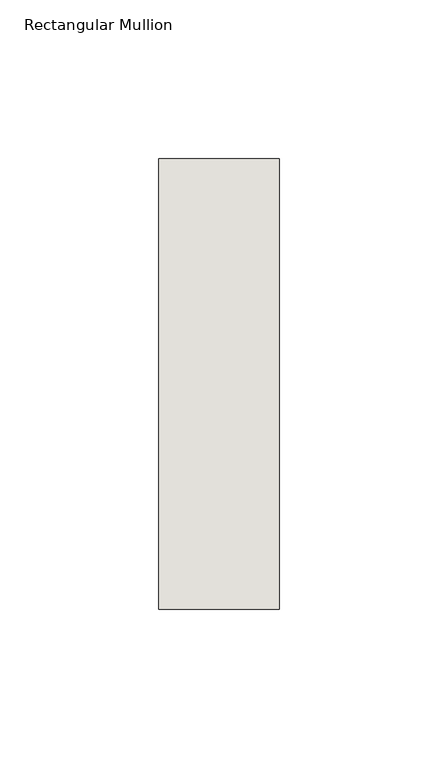
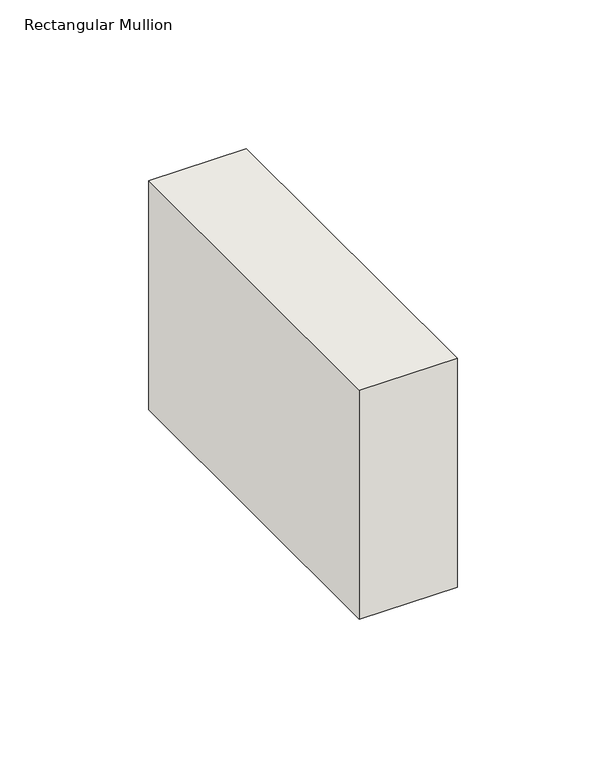
"""IFC4 building model written with IfcOpenShell, lengths in millimetres: wall geometry, Rectangular Mullion : NLRS_21_CWM_hsb-regel 38x142_gen_rsf."""

from ifc_helpers import new_model, si_unit, frame, origin, place, context, project, spatial, polyline, outline, extrude, source, transform, mapped, element, save


def rectangular_mullion_ff2f71bd(model_context):
    return source(origin(), model_context, "Body", "SweptSolid", [
        extrude(outline(polyline([(0.0, -71.0), (-38.0, -71.0), (-38.0, 71.0), (0.0, 71.0), (0.0, -71.0)])), frame((0.0, 0.0, -94.1558939), z_axis=(0.0, 0.0, 1.0), x_axis=(1.0, 0.0, 0.0)), (0.0, 0.0, 1.0), 94.1558939),
    ])


if __name__ == "__main__":
    model = new_model("IFC4")
    model_context = context("Model", 3, world=origin())
    ifc_project = project(units=[si_unit("LENGTHUNIT", "METRE", prefix="MILLI")], contexts=[model_context])
    site = spatial("IfcSite", under=ifc_project)
    building = spatial("IfcBuilding", under=site)
    placement = place(None, origin())
    rectangular_mullion_shape = rectangular_mullion_ff2f71bd(model_context)
    element("IfcWall", 1, ObjectType="Rectangular Mullion : NLRS_21_CWM_hsb-regel 38x142_gen_rsf", at=placement, inside=building, context=model_context, shape_type="MappedRepresentation", body=[
        mapped(rectangular_mullion_shape, transform((0.0, 0.0, 0.0), x_axis=(1.0, 0.0, 0.0), y_axis=(0.0, 1.0, 0.0), z_axis=(0.0, 0.0, 1.0))),
    ])
    save(model, "model.ifc")

# Revit data of these elements
# Type "Rectangular Mullion : NLRS_21_CWM_hsb-regel 38x142_gen_rsf"
#   Type IfcGUID = "07M7mRoiH1CR8m_RSKIwpF"
#   Assembly Code = "21.10"
#   IfcExportAs = "IfcWall"
#   built-in parameter 1007322 = 0.465879 (stored number, unit not read)
#   built-in parameter 1007321 = 0.062336 (stored number, unit not read)
#   built-in parameter 1007320 = 0.062336 (stored number, unit not read)
# Element 1 (IfcWall, "Rectangular Mullion : NLRS_21_CWM_hsb-regel 38x142_gen_rsf")
#   Materials on its faces: "NLRS_i2_hout naaldhout vuren_gen_rsf"
# Materials
#   "NLRS_i2_hout naaldhout vuren_gen_rsf": class "I - Hout", colour RGB 234 199 147, transparency 0, Keynote = "i2", Manufacturer = "Revit Standards Foundation", URL = "www.revitstandards.org", Description = "hout vuren", Cost = 0
